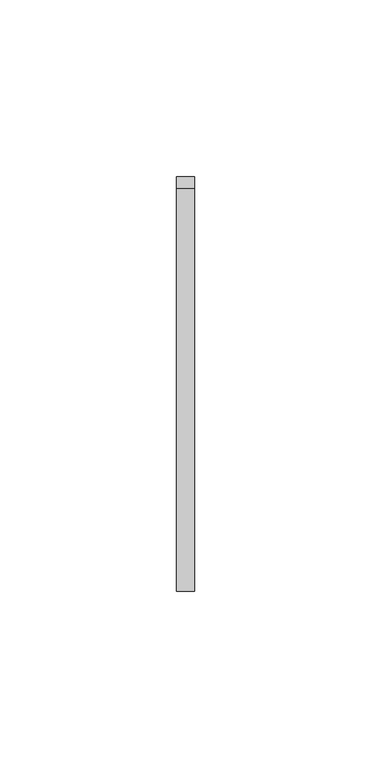
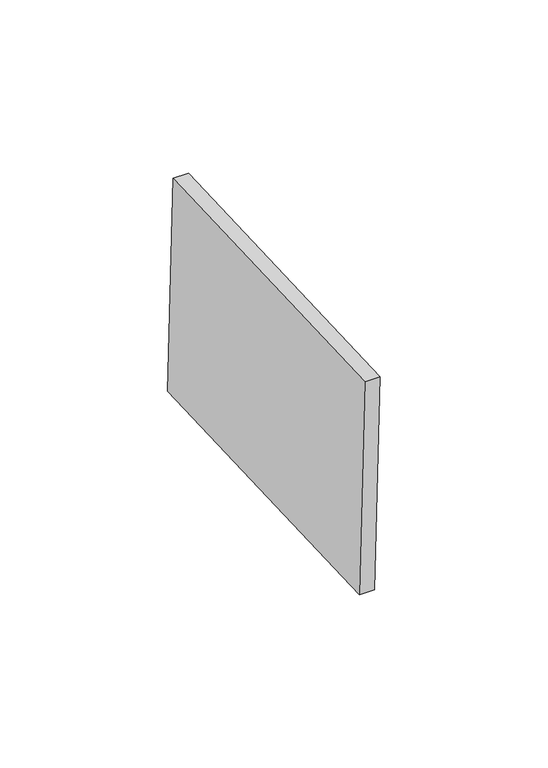
"""IFC4 building model written with IfcOpenShell, lengths in millimetres: proxy geometry, Inner panel:Inner panel:1:Inner panel:1 : Inner panel:Inner panel:300324:2:Inner panel:1:Inner panel:1 : Inner panel:Inner panel:300324:2 : Inner panel:Inner panel:1:Inner panel:1 : Inner panel:Inner panel:300324:300043:23 : Inner panel:Inner panel:1:Inner panel:1 : Inner panel:Inner panel:300324:2:Inner panel:1:Inner panel:1 : Inner panel:Inner panel:300324:2 : Inner panel:Inner panel:1:Inner panel:1 : Inner panel:Inner panel:300324:300043:308120."""

import ifcopenshell
import ifcopenshell.guid

model = None  # the IFC model being written
_history = None  # IfcOwnerHistory: only IFC2X3 demands one
_inside = {}  # id of a spatial element -> (the spatial element, [elements in it])
_under = {}  # id of a project, library or spatial element -> (it, [spatial elements below it])
_declared = {}  # id of a project -> (the project, [libraries it declares])
_typed = {}  # id of a type object -> (the type object, [elements of that type])
_made_of = {}  # id of a material, layer set ... -> (it, [elements and type objects made of it])


def new_model(schema):
    """Start an empty IFC model of exactly this schema.

    Asked for "IFC4X3", IfcOpenShell would pick the latest addendum, in which some entities
    have other attributes; the version numbers below select the first issue.
    IFC2X3 requires an IfcOwnerHistory on every rooted entity: one is made here for all.
    """
    global model, _history
    if schema == "IFC4X3":
        model = ifcopenshell.file(schema_version=(4, 3, 0, 0))
    else:
        model = ifcopenshell.file(schema=schema)
    _inside.clear()
    _under.clear()
    _declared.clear()
    _typed.clear()
    _made_of.clear()
    _history = None
    if model.schema == "IFC2X3":
        org = make("IfcOrganization", Name="unknown")
        user = make(
            "IfcPersonAndOrganization",
            ThePerson=make("IfcPerson", FamilyName="unknown"),
            TheOrganization=org,
        )
        app = make(
            "IfcApplication",
            ApplicationDeveloper=org,
            Version="unknown",
            ApplicationFullName="unknown",
            ApplicationIdentifier="unknown",
        )
        _history = make(
            "IfcOwnerHistory",
            OwningUser=user,
            OwningApplication=app,
            ChangeAction="ADDED",
            CreationDate=0,
        )
    return model


def make(cls, **values):
    """One entity of the class cls with the attributes given. An attribute that is None is left unset."""
    return model.create_entity(
        cls, **{name: value for name, value in values.items() if value is not None}
    )


def rooted(cls, **values):
    """An entity with a GlobalId (a new one), such as an element, a storey or a relation."""
    return make(cls, GlobalId=ifcopenshell.guid.new(), OwnerHistory=_history, **values)


def si_unit(unit_type, name, prefix=None):
    """IfcSIUnit, for example si_unit("LENGTHUNIT", "METRE", prefix="MILLI")."""
    return make("IfcSIUnit", UnitType=unit_type, Prefix=prefix, Name=name)


def assignment(units):
    """IfcUnitAssignment: the units of a project."""
    return None if units is None else make("IfcUnitAssignment", Units=units)


def point(xyz):
    """IfcCartesianPoint."""
    return None if xyz is None else make("IfcCartesianPoint", Coordinates=xyz)


def direction(xyz):
    """IfcDirection."""
    return None if xyz is None else make("IfcDirection", DirectionRatios=xyz)


def frame(location, z_axis=None, x_axis=None):
    """IfcAxis2Placement3D, a coordinate frame: its origin and axes. An axis left out is left unset."""
    return make(
        "IfcAxis2Placement3D",
        Location=point(location),
        Axis=direction(z_axis),
        RefDirection=direction(x_axis),
    )


def origin():
    """The frame at (0, 0, 0) with its axes left unset."""
    return frame((0.0, 0.0, 0.0))


def place(relative_to, where):
    """IfcLocalPlacement: puts the frame where relative to a parent placement (None: the world)."""
    return make(
        "IfcLocalPlacement", PlacementRelTo=relative_to, RelativePlacement=where
    )


def context(
    kind, dimensions, precision=None, world=None, true_north=None, identifier=None
):
    """IfcGeometricRepresentationContext, for example the 3D "Model" context."""
    return make(
        "IfcGeometricRepresentationContext",
        ContextIdentifier=identifier,
        ContextType=kind,
        CoordinateSpaceDimension=dimensions,
        Precision=precision,
        WorldCoordinateSystem=world,
        TrueNorth=true_north,
    )


def project(units=None, contexts=None):
    """IfcProject with its units and contexts."""
    return rooted(
        "IfcProject",
        Name="project",
        RepresentationContexts=contexts,
        UnitsInContext=assignment(units),
    )


def spatial(cls, under=None, at=None, **own):
    """A site, building, storey or space (cls), placed at a placement, below another one or the project."""
    s = rooted(cls, ObjectPlacement=at, **own)
    if under is not None:
        _under.setdefault(under.id(), (under, []))[1].append(s)
    return s


def polyline(points):
    """IfcPolyline through the points."""
    return make("IfcPolyline", Points=[point(p) for p in points])


def outline(outer, holes=None, kind="AREA"):
    """IfcArbitraryClosedProfileDef: a profile drawn as a closed curve; with holes, ...WithVoids."""
    if holes is None:
        return make("IfcArbitraryClosedProfileDef", ProfileType=kind, OuterCurve=outer)
    return make(
        "IfcArbitraryProfileDefWithVoids",
        ProfileType=kind,
        OuterCurve=outer,
        InnerCurves=holes,
    )


def extrude(swept, where, along, depth):
    """IfcExtrudedAreaSolid: the profile swept, set in the frame where, extruded along a direction by depth."""
    return make(
        "IfcExtrudedAreaSolid",
        SweptArea=swept,
        Position=where,
        ExtrudedDirection=direction(along),
        Depth=depth,
    )


def shape(context_of_items, identifier, shape_type, items):
    """IfcShapeRepresentation: the items that make up one representation, for example the "Body"."""
    return make(
        "IfcShapeRepresentation",
        ContextOfItems=context_of_items,
        RepresentationIdentifier=identifier,
        RepresentationType=shape_type,
        Items=items,
    )


def source(mapping_origin, context_of_items, identifier, shape_type, items):
    """IfcRepresentationMap: a shape defined once, which mapped items show again and again."""
    return make(
        "IfcRepresentationMap",
        MappingOrigin=mapping_origin,
        MappedRepresentation=shape(context_of_items, identifier, shape_type, items),
    )


def transform(
    local_origin,
    x_axis=None,
    y_axis=None,
    z_axis=None,
    scale=None,
    scale2=None,
    scale3=None,
    uniform=True,
):
    """IfcCartesianTransformationOperator3D, or its non-uniform kind. x_axis, y_axis, z_axis: its Axis1, 2, 3."""
    if uniform:
        return make(
            "IfcCartesianTransformationOperator3D",
            Axis1=direction(x_axis),
            Axis2=direction(y_axis),
            LocalOrigin=point(local_origin),
            Scale=scale,
            Axis3=direction(z_axis),
        )
    return make(
        "IfcCartesianTransformationOperator3DnonUniform",
        Axis1=direction(x_axis),
        Axis2=direction(y_axis),
        LocalOrigin=point(local_origin),
        Scale=scale,
        Axis3=direction(z_axis),
        Scale2=scale2,
        Scale3=scale3,
    )


def mapped(mapping_source, mapping_target):
    """IfcMappedItem: shows the shape of a source again, moved by a transform."""
    return make(
        "IfcMappedItem", MappingSource=mapping_source, MappingTarget=mapping_target
    )


def made_of(thing, what):
    """Note that an element or type object is made of a material, layer set ...; save() writes the relation."""
    if what is not None:
        _made_of.setdefault(what.id(), (what, []))[1].append(thing)
    return thing


def element(
    cls,
    number,
    at=None,
    inside=None,
    cuts=None,
    type_object=None,
    material=None,
    context=None,
    identifier="Body",
    shape_type=None,
    held_by="IfcProductDefinitionShape",
    body=None,
    shapes=None,
    **own,
):
    """One element of the class cls, such as IfcWall. Its Tag is "e" and its number.

    at: its placement. inside: the storey or other place that contains it. cuts: it is an
    opening in that element (IfcRelVoidsElement). A single representation is given by context,
    identifier, shape_type and body (its items); several are given by shapes. held_by: the class
    of the entity that holds the representations. save() writes the other relations.
    """
    e = rooted(cls, Tag="e%d" % number, ObjectPlacement=at, **own)
    if body is not None:
        shapes = [shape(context, identifier, shape_type, body)]
    if shapes is not None:
        e.Representation = make(held_by, Representations=shapes)
    if inside is not None:
        _inside.setdefault(inside.id(), (inside, []))[1].append(e)
    if cuts is not None:
        rooted(
            "IfcRelVoidsElement", RelatingBuildingElement=cuts, RelatedOpeningElement=e
        )
    if type_object is not None:
        _typed.setdefault(type_object.id(), (type_object, []))[1].append(e)
    return made_of(e, material)


def aggregate(whole, parts):
    """IfcRelAggregates: a whole, such as a stair, and the parts it consists of."""
    return rooted("IfcRelAggregates", RelatingObject=whole, RelatedObjects=parts)


def save(model, path):
    """Write the relations noted so far, then the file.

    IfcRelAggregates (storeys below a building ...), IfcRelContainedInSpatialStructure (elements
    in a storey), IfcRelDefinesByType, IfcRelAssociatesMaterial and IfcRelDeclares: one each for
    every whole, place, type object, material and project.
    """
    for whole, parts in _under.values():
        aggregate(whole, parts)
    for where, things in _inside.values():
        rooted(
            "IfcRelContainedInSpatialStructure",
            RelatedElements=things,
            RelatingStructure=where,
        )
    for kind, things in _typed.values():
        rooted("IfcRelDefinesByType", RelatedObjects=things, RelatingType=kind)
    for what, things in _made_of.values():
        rooted("IfcRelAssociatesMaterial", RelatedObjects=things, RelatingMaterial=what)
    for by, libraries in _declared.values():
        rooted("IfcRelDeclares", RelatingContext=by, RelatedDefinitions=libraries)
    model.write(path)


def generic_models_54825b19(model_context):
    return source(origin(), model_context, "Body", "SweptSolid", [
        extrude(outline(polyline([(0.0, -114.3), (0.0, 0.0), (5.2138089, 0.0), (5.2138089, -114.3), (0.0, -114.3)])), frame((593530.195117, -564692.6498794, 8923.8568948), z_axis=(0.0, -0.04163054471218449, 0.9991330730923519), x_axis=(-1.0, 0.0, 0.0)), (0.0, 0.0, 1.0), 79.375),
    ])


if __name__ == "__main__":
    model = new_model("IFC4")
    model_context = context("Model", 3, world=origin())
    ifc_project = project(units=[si_unit("LENGTHUNIT", "METRE", prefix="MILLI")], contexts=[model_context])
    site = spatial("IfcSite", under=ifc_project)
    building = spatial("IfcBuilding", under=site)
    placement = place(None, origin())
    generic_models_shape = generic_models_54825b19(model_context)
    element("IfcBuildingElementProxy", 1, Name="Inner panel:Inner panel:1:Inner panel:1 : Inner panel:Inner panel:300324:2:Inner panel:1:Inner panel:1 : Inner panel:Inner panel:300324:2 : Inner panel:Inner panel:1:Inner panel:1 : Inner panel:Inner panel:300324:300043:23 : Inner panel:Inner panel:1:Inner panel:1 : Inner panel:Inner panel:300324:2:Inner panel:1:Inner panel:1 : Inner panel:Inner panel:300324:2 : Inner panel:Inner panel:1:Inner panel:1 : Inner panel:Inner panel:300324:300043:308120", ObjectType="Inner panel:Inner panel:1:Inner panel:1 : Inner panel:Inner panel:300324:2:Inner panel:1:Inner panel:1 : Inner panel:Inner panel:300324:2 : Inner panel:Inner panel:1:Inner panel:1 : Inner panel:Inner panel:300324:300043:23 : Inner panel:Inner panel:1:Inner panel:1 : Inner panel:Inner panel:300324:2:Inner panel:1:Inner panel:1 : Inner panel:Inner panel:300324:2 : Inner panel:Inner panel:1:Inner panel:1 : Inner panel:Inner panel:300324:300043:308120", at=placement, inside=building, context=model_context, shape_type="MappedRepresentation", body=[
        mapped(generic_models_shape, transform((0.0, 0.0, 0.0), x_axis=(1.0, 0.0, 0.0), y_axis=(0.0, 1.0, 0.0), z_axis=(0.0, 0.0, 1.0))),
    ])
    save(model, "model.ifc")

# Revit data of these elements
# Type "Inner panel:Inner panel:1:Inner panel:1 : Inner panel:Inner panel:300324:2:Inner panel:1:Inner panel:1 : Inner panel:Inner panel:300324:2 : Inner panel:Inner panel:1:Inner panel:1 : Inner panel:Inner panel:300324:300043:23 : Inner panel:Inner panel:1:Inner panel:1 : Inner panel:Inner panel:300324:2:Inner panel:1:Inner panel:1 : Inner panel:Inner panel:300324:2 : Inner panel:Inner panel:1:Inner panel:1 : Inner panel:Inner panel:300324:300043:308120"
#   NameOverride = "Inner panel:Inner panel:1:Inner panel:1 : Inner panel:Inner panel:300324:2:Inner panel:1:Inner panel:1 : Inner panel:Inner panel:300324:2 : Inner panel:Inner panel:1:Inner panel:1 : Inner panel:Inner panel:300324:300043:308120"
#   ObjectTypeOverride = "Inner panel:1:Inner panel:1 : Inner panel:Inner panel:300324:2 : Inner panel:Inner panel:1:Inner panel:1 : Inner panel:Inner panel:300324:300043"
#   Reference = "Inner panel"
#   Tag = "308120"
# Element 1 (IfcBuildingElementProxy, "Inner panel:Inner panel:1:Inner panel:1 : Inner panel:Inner panel:300324:2:Inner panel:1:Inner panel:1 : Inner panel:Inner panel:300324:2 : Inner panel:Inner panel:1:Inner panel:1 : Inner panel:Inner panel:300324:300043:23 : Inner panel:Inner panel:1:Inner panel:1 : Inner panel:Inner panel:300324:2:Inner panel:1:Inner panel:1 : Inner panel:Inner panel:300324:2 : Inner panel:Inner panel:1:Inner panel:1 : Inner panel:Inner panel:300324:300043:308120")
#   Materials on its faces: "SLIDING CLIP"
# Materials
#   "SLIDING CLIP": class "Generic", colour RGB 120 120 120, transparency 0, Cost = 0
